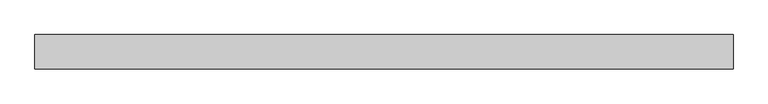
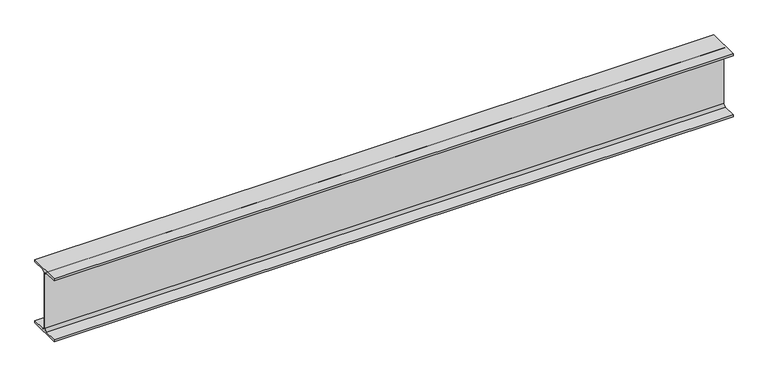
"""IFC4 building model written with IfcOpenShell, lengths in millimetres: beam geometry, 0912_Steel Framing_H-KSD3502 : H_SB_AR_S02_H-350x175x7x11_Platform."""

from ifc_helpers import new_model, si_unit, point, frame, frame_2d, origin, place, context, project, spatial, polyline, circle_curve, trimmed, segment, composite_curve, outline, extrude, source, transform, mapped, element, save


def beam_edcef29c(model_context):
    return source(origin(), model_context, "Body", "SweptSolid", [
        extrude(outline(composite_curve([segment(polyline([(87.5, -164.0), (87.5, -175.0), (-87.5, -175.0), (-87.5, -164.0), (-17.5, -164.0)]), True, "CONTINUOUS"), segment(trimmed(circle_curve(frame_2d((-17.5, -150.0)), 14.0), [point((-17.5, -164.0))], [point((-3.5, -150.0))], True, "CARTESIAN"), True, "CONTINUOUS"), segment(polyline([(-3.5, -150.0), (-3.5, 150.0)]), True, "CONTINUOUS"), segment(trimmed(circle_curve(frame_2d((-17.5, 150.0)), 14.0), [point((-3.5, 150.0))], [point((-17.5, 164.0))], True, "CARTESIAN"), True, "CONTINUOUS"), segment(polyline([(-17.5, 164.0), (-87.5, 164.0), (-87.5, 175.0), (87.5, 175.0), (87.5, 164.0), (17.5, 164.0)]), True, "CONTINUOUS"), segment(trimmed(circle_curve(frame_2d((17.5, 150.0)), 14.0), [point((17.5, 164.0))], [point((3.5, 150.0))], True, "CARTESIAN"), True, "CONTINUOUS"), segment(polyline([(3.5, 150.0), (3.5, -150.0)]), True, "CONTINUOUS"), segment(trimmed(circle_curve(frame_2d((17.5, -150.0)), 14.0), [point((3.5, -150.0))], [point((17.5, -164.0))], True, "CARTESIAN"), True, "CONTINUOUS"), segment(polyline([(17.5, -164.0), (87.5, -164.0)]), True, "CONTINUOUS")], self_intersect=False)), frame((-1787.3, 0.0, 0.0), z_axis=(1.0, 0.0, 0.0), x_axis=(0.0, 1.0, 0.0)), (0.0, 0.0, 1.0), 3574.6),
    ])


if __name__ == "__main__":
    model = new_model("IFC4")
    model_context = context("Model", 3, world=origin())
    ifc_project = project(units=[si_unit("LENGTHUNIT", "METRE", prefix="MILLI")], contexts=[model_context])
    site = spatial("IfcSite", under=ifc_project)
    building = spatial("IfcBuilding", under=site)
    placement = place(None, origin())
    beam_shape = beam_edcef29c(model_context)
    element("IfcBeam", 1, ObjectType="0912_Steel Framing_H-KSD3502 : H_SB_AR_S02_H-350x175x7x11_Platform", at=placement, inside=building, context=model_context, shape_type="MappedRepresentation", body=[
        mapped(beam_shape, transform((0.0, 0.0, 0.0), x_axis=(1.0, 0.0, 0.0), y_axis=(0.0, 1.0, 0.0), z_axis=(0.0, 0.0, 1.0))),
    ])
    save(model, "model.ifc")

# Revit data of these elements
# Type "0912_Steel Framing_H-KSD3502 : H_SB_AR_S02_H-350x175x7x11_Platform"
#   H_Q'ty Cal Type Tag = "SB-Q2"
#   H_WM Code_1 = "S01AA073-00001 |  | TON | Main Steel Structure Fabrication Work | Shelter/Building | Medium Steel - Standard |  |  |  |  |  |  | Material: (   ) | (90)KG/M>Weight≥(30)KG/M | S01AA073-00001 Main Steel Structure Fabrication Work Shelter/Building Medium Steel - Standard         | - Material: ( ASTM A36 )\n- (90)KG/M>Weight≥(30)KG/M"
#   H_WM Code_2 = "S03AA083-00001 |  | TON | Main Steel Structure Erection Work | Shelter/Building | Medium Steel |  |  |  |  |  |  | Material: (   ) | S03AA083-00001 Main Steel Structure Erection Work Shelter/Building Medium Steel         | - Material: ( ASTM A36 )"
#   H_WM Code_3 = "S01AA009-00001 |  | TON | Main Steel Structure Fabrication Work | Shelter/Building | Plates - Gusset, Stiffener, ETC | Material: (   ) | S01AA009-00001 Main Steel Structure Fabrication Work Shelter/Building Plates - Gusset, Stiffener, ETC         |"
#   H_WM Code_4 = "S41AA051-00001 |  | M2 | Steel Structure Paint Work | Shelter/Building | for Non-Fireproofed Steel Surface |  |  |  |  |  |  | Material: (   ) | S41AA051-00001 Steel Structure Paint Work Shelter/Building for Non-Fireproofed Steel Surface         |"
#   Width = 17.5 cm
#   Web Thickness = 0.7 cm
#   Web Fillet = 1.4 cm
#   Warping Constant = 282000.0 cm⁶
#   W = 0
#   Torsional Moment of Inertia = 19.4042 cm⁴
#   Section Area = 63.14 cm²
#   Plastic Modulus weak axis = 174.0 cm³
#   Plastic Modulus strong axis = 868.0 cm³
#   Perimeter = 1.36 m²/m
#   Nominal Weight = 49.60 kgf/m
#   Moment of Inertia weak axis = 984.00 cm⁴
#   Moment of Inertia strong axis = 13600.00 cm⁴
#   Height = 35.0 cm
#   Flange Thickness = 1.1 cm
#   Elastic Modulus weak axis = 112.0 cm³
#   Elastic Modulus strong axis = 775.0 cm³
#   Centroid Vertical = 17.5 cm
#   Centroid Horizontal = 8.75 cm
#   Ix = 136000000
#   Length [instance default] = 1524 mm
#   Zx = 868000
#   b = 175 mm
#   h = 350 mm
#   r = 14 mm
#   s = 7 mm
#   t = 11 mm
#   A = 0.006314 m²
#   Structural Material [instance default] = Steel, 45-345
#   Assembly Code = ""
# Element 1 (IfcBeam, "0912_Steel Framing_H-KSD3502 : H_SB_AR_S02_H-350x175x7x11_Platform")
#   Materials on its faces: "Steel, 45-345"
# Materials
#   "Steel, 45-345": class "Metal", colour RGB 189 187 185, transparency 0, Description = "Steel 345 MPa", Cost = 0
